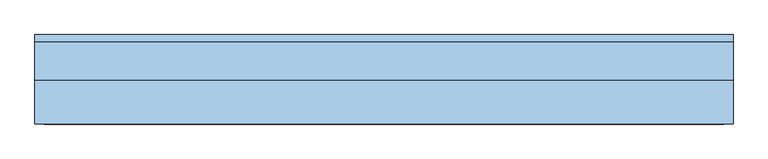
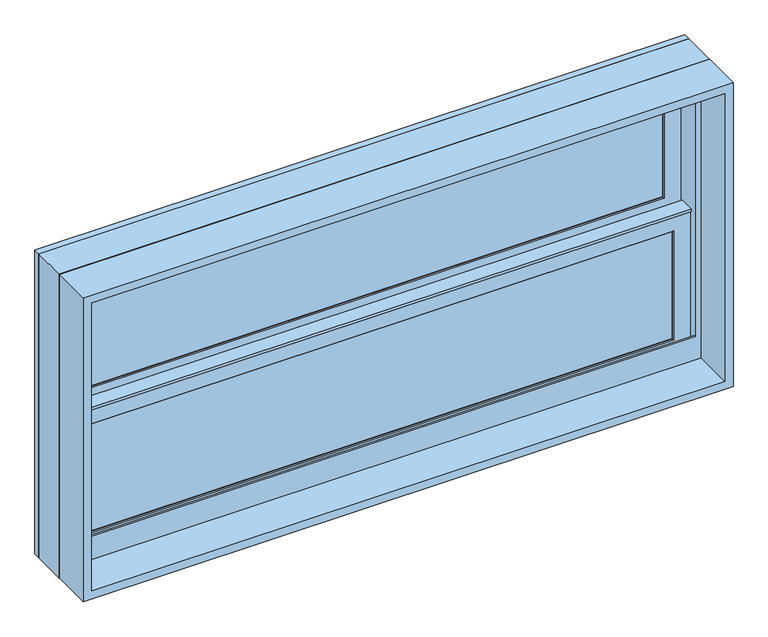
"""IFC4 building model written with IfcOpenShell, lengths in millimetres: window geometry, Window-Double_Hung-Marvin-Essential : ESDH4020."""

from ifc_helpers import new_model, si_unit, frame, origin, place, context, project, spatial, polyline, outline, extrude, faceted_brep, source, transform, mapped, element, save


def window_6a7649f0(model_context):
    return source(origin(), model_context, "Body", "SolidModel", [
        extrude(outline(polyline([(191.5583333, 20.6375), (191.5583333, 15.875), (172.5083333, 15.875), (172.5083333, 20.6375), (191.5583333, 20.6375)])), frame((0.0, 0.0, 1898.65), z_axis=(0.0, 0.0, 1.0), x_axis=(1.0, 0.0, 0.0)), (0.0, 0.0, 1.0), 222.25),
        extrude(outline(polyline([(-172.5083333, 20.6375), (-172.5083333, 15.875), (-191.5583333, 15.875), (-191.5583333, 20.6375), (-172.5083333, 20.6375)])), frame((0.0, 0.0, 1898.65), z_axis=(0.0, 0.0, 1.0), x_axis=(1.0, 0.0, 0.0)), (0.0, 0.0, 1.0), 222.25),
        extrude(outline(polyline([(546.1, 20.6375), (546.1, 15.875), (-546.1, 15.875), (-546.1, 20.6375), (546.1, 20.6375)])), frame((0.0, 0.0, 2000.25), z_axis=(0.0, 0.0, 1.0), x_axis=(1.0, 0.0, 0.0)), (0.0, 0.0, 1.0), 19.05),
        extrude(outline(polyline([(-191.5583333, 46.83125), (-191.5583333, 51.59375), (-172.5083333, 51.59375), (-172.5083333, 46.83125), (-191.5583333, 46.83125)])), frame((0.0, 0.0, 2159.0), z_axis=(0.0, 0.0, 1.0), x_axis=(1.0, 0.0, 0.0)), (0.0, 0.0, 1.0), 222.25),
        extrude(outline(polyline([(172.5083333, 46.83125), (172.5083333, 51.59375), (191.5583333, 51.59375), (191.5583333, 46.83125), (172.5083333, 46.83125)])), frame((0.0, 0.0, 2159.0), z_axis=(0.0, 0.0, 1.0), x_axis=(1.0, 0.0, 0.0)), (0.0, 0.0, 1.0), 222.25),
        extrude(outline(polyline([(-546.1, 46.83125), (-546.1, 51.59375), (546.1, 51.59375), (546.1, 46.83125), (-546.1, 46.83125)])), frame((0.0, 0.0, 2260.6), z_axis=(0.0, 0.0, 1.0), x_axis=(1.0, 0.0, 0.0)), (0.0, 0.0, 1.0), 19.05),
        extrude(outline(polyline([(191.5583333, 20.6375), (172.5083333, 20.6375), (172.5083333, 25.4), (191.5583333, 25.4), (191.5583333, 20.6375)])), frame((0.0, 0.0, 1898.65), z_axis=(0.0, 0.0, 1.0), x_axis=(1.0, 0.0, 0.0)), (0.0, 0.0, 1.0), 222.25),
        extrude(outline(polyline([(-172.5083333, 20.6375), (-191.5583333, 20.6375), (-191.5583333, 25.4), (-172.5083333, 25.4), (-172.5083333, 20.6375)])), frame((0.0, 0.0, 1898.65), z_axis=(0.0, 0.0, 1.0), x_axis=(1.0, 0.0, 0.0)), (0.0, 0.0, 1.0), 222.25),
        extrude(outline(polyline([(546.1, 20.6375), (-546.1, 20.6375), (-546.1, 25.4), (546.1, 25.4), (546.1, 20.6375)])), frame((0.0, 0.0, 2000.25), z_axis=(0.0, 0.0, 1.0), x_axis=(1.0, 0.0, 0.0)), (0.0, 0.0, 1.0), 19.05),
        extrude(outline(polyline([(-191.5583333, 56.35625), (-172.5083333, 56.35625), (-172.5083333, 51.59375), (-191.5583333, 51.59375), (-191.5583333, 56.35625)])), frame((0.0, 0.0, 2159.0), z_axis=(0.0, 0.0, 1.0), x_axis=(1.0, 0.0, 0.0)), (0.0, 0.0, 1.0), 222.25),
        extrude(outline(polyline([(172.5083333, 56.35625), (191.5583333, 56.35625), (191.5583333, 51.59375), (172.5083333, 51.59375), (172.5083333, 56.35625)])), frame((0.0, 0.0, 2159.0), z_axis=(0.0, 0.0, 1.0), x_axis=(1.0, 0.0, 0.0)), (0.0, 0.0, 1.0), 222.25),
        extrude(outline(polyline([(-546.1, 56.35625), (546.1, 56.35625), (546.1, 51.59375), (-546.1, 51.59375), (-546.1, 56.35625)])), frame((0.0, 0.0, 2260.6), z_axis=(0.0, 0.0, 1.0), x_axis=(1.0, 0.0, 0.0)), (0.0, 0.0, 1.0), 19.05),
        faceted_brep([(-573.0875, 5.6780605, 2150.9351748), (-573.0875, 5.6780605, 2146.3), (573.0875, 5.6780605, 2146.3), (573.0875, 5.6780605, 2150.9351748), (-573.0875, 34.8118605, 2150.9351748), (573.0875, 34.8118605, 2150.9351748), (573.0875, 34.8118605, 2146.3), (-573.0875, 34.8118605, 2146.3), (-573.0875, 30.1625, 2146.3), (-573.0875, 30.1625, 1871.6625), (-573.0875, 8.9241104, 1871.6625), (-573.0875, 8.9241104, 2146.3), (573.0875, 8.9241104, 2146.3), (573.0875, 30.1625, 2146.3), (573.0875, 8.9241104, 1871.6625), (573.0875, 30.1625, 1871.6625), (-557.2034752, 11.90625, 2132.0034752), (-557.2034752, 30.1625, 2132.0034752), (557.2034752, 30.1625, 2132.0034752), (557.2034752, 11.90625, 2132.0034752), (-540.54375, 10.4662439, 2115.34375), (-540.54375, 11.90625, 2115.34375), (540.54375, 11.90625, 2115.34375), (540.54375, 10.4662439, 2115.34375), (542.0858834, 8.9241104, 2116.8858834), (-542.0858834, 8.9241104, 2116.8858834), (557.2034752, 30.1625, 1887.5465248), (557.2034752, 11.90625, 1887.5465248), (540.54375, 11.90625, 1904.20625), (540.54375, 10.4662439, 1904.20625), (542.0858834, 8.9241104, 1902.6641166), (-557.2034752, 30.1625, 1887.5465248), (-557.2034752, 11.90625, 1887.5465248), (-540.54375, 11.90625, 1904.20625), (-540.54375, 10.4662439, 1904.20625), (-542.0858834, 8.9241104, 1902.6641166)], [[[0, 1, 2, 3]], [[4, 5, 6, 7]], [[1, 0, 4, 7, 8, 9, 10, 11]], [[2, 1, 11, 12]], [[7, 6, 13, 8]], [[3, 2, 12, 14, 15, 13, 6, 5]], [[0, 3, 5, 4]], [[16, 17, 18, 19]], [[20, 21, 22, 23]], [[20, 23, 24, 25]], [[19, 18, 26, 27]], [[23, 22, 28, 29]], [[24, 23, 29, 30]], [[27, 26, 31, 32]], [[29, 28, 33, 34]], [[30, 29, 34, 35]], [[15, 14, 10, 9]], [[15, 9, 8, 13], [18, 17, 31, 26]], [[17, 16, 32, 31]], [[16, 19, 27, 32], [22, 21, 33, 28]], [[21, 20, 34, 33]], [[20, 25, 35, 34]], [[10, 14, 12, 11], [25, 24, 30, 35]]]),
        extrude(outline(polyline([(38.5955581, 2132.0125), (33.5778968, 2132.0125), (33.5778968, 2133.6), (39.9405976, 2133.6), (39.9405976, 2132.0125), (61.515625, 2132.0125), (47.6307501, 2128.6975159), (38.5955581, 2128.6975159), (38.5955581, 2132.0125)])), frame((-573.0875, 0.0, 0.0), z_axis=(1.0, 0.0, 0.0), x_axis=(0.0, 1.0, 0.0)), (0.0, 0.0, 1.0), 1146.175),
        faceted_brep([(603.25, 0.0, 1841.5), (603.25, 0.0, 2438.4), (-603.25, 0.0, 2438.4), (-603.25, 0.0, 1841.5), (577.05625, 0.0, 1902.61875), (-577.05625, 0.0, 1902.61875), (-577.05625, 0.0, 2412.20625), (577.05625, 0.0, 2412.20625), (577.05625, 3.96875, 1841.5), (-577.05625, 3.96875, 1841.5), (-577.05625, 3.96875, 1902.61875), (577.05625, 3.96875, 1902.61875), (-603.25, 65.6828125, 1841.5), (-577.05625, 65.6828125, 1841.5), (577.05625, 65.6828125, 1841.5), (603.25, 65.6828125, 1841.5), (-603.25, 65.6828125, 2438.4), (603.25, 65.6828125, 2438.4), (577.05625, 65.6828125, 2412.20625), (-577.05625, 65.6828125, 2412.20625)], [[[0, 1, 2, 3], [4, 5, 6, 7]], [[8, 9, 10, 11]], [[5, 4, 11, 10]], [[0, 3, 12, 13, 9, 8, 14, 15]], [[13, 12, 16, 17, 15, 14, 18, 19]], [[13, 19, 6, 5, 10, 9]], [[7, 6, 19, 18]], [[18, 14, 8, 11, 4, 7]], [[1, 0, 15, 17]], [[2, 1, 17, 16]], [[3, 2, 16, 12]]]),
        faceted_brep([(577.05625, 30.1625, 2139.95), (575.46875, 30.1625, 2139.95), (575.46875, 30.1625, 1865.8544613), (577.05625, 30.1625, 1865.8544613), (-575.46875, 30.1625, 2139.95), (-577.05625, 30.1625, 2139.95), (-577.05625, 30.1625, 1865.8544613), (-575.46875, 30.1625, 1865.8544613), (575.46875, 63.5, 2139.95), (577.05625, 63.5, 2139.95), (577.05625, 63.5, 1859.3743077), (575.46875, 63.5, 1859.3743077), (-577.05625, 63.5, 2139.95), (-575.46875, 63.5, 2139.95), (-575.46875, 63.5, 1859.3743077), (-577.05625, 63.5, 1859.3743077), (588.3108932, 3.96875, 1870.9460105), (588.3108932, 3.96875, 1841.5), (588.3108932, 65.6828125, 1841.5), (588.3108932, 65.6828125, 1858.950012), (-588.3108932, 3.96875, 1841.5), (-588.3108932, 3.96875, 1870.9460105), (-588.3108932, 65.6828125, 1858.950012), (-588.3108932, 65.6828125, 1841.5), (588.3108932, 78.58125, 1856.4428097), (-588.3108932, 78.58125, 1856.4428097), (-586.2971252, 68.2348864, 1858.4539391), (-568.33135, 68.2348864, 1858.4539391), (-568.33135, 65.6828125, 1858.950012), (568.33135, 65.6828125, 1858.950012), (568.33135, 68.2348864, 1858.4539391), (586.2971252, 68.2348864, 1858.4539391), (-603.25, 65.6828125, 1841.5), (-603.25, 78.5948249, 1841.5), (603.25, 78.5948249, 1841.5), (603.25, 65.6828125, 1841.5), (-603.25, 78.58125, 2438.4), (603.25, 78.58125, 2438.4), (588.3108932, 78.58125, 2423.4608932), (-588.3108932, 78.58125, 2423.4608932), (-603.25, 65.6828125, 2438.4), (-586.2971252, 68.2348864, 2421.4471252), (586.2971252, 68.2348864, 2421.4471252), (568.33135, 68.2348864, 2403.48135), (-568.33135, 68.2348864, 2403.48135), (-568.33135, 65.6828125, 2403.48135), (568.33135, 65.6828125, 2403.48135), (603.25, 65.6828125, 2438.4)], [[[0, 1, 2, 3]], [[4, 5, 6, 7]], [[8, 9, 10, 11]], [[12, 13, 14, 15]], [[1, 8, 11, 2]], [[9, 0, 3, 10]], [[1, 0, 9, 8]], [[5, 4, 13, 12]], [[5, 12, 15, 6]], [[13, 4, 7, 14]], [[16, 17, 18, 19]], [[20, 21, 22, 23]], [[24, 25, 26, 27, 28, 22, 21, 16, 19, 29, 30, 31], [3, 2, 11, 10], [7, 6, 15, 14]], [[17, 16, 21, 20]], [[17, 20, 23, 32, 33, 34, 35, 18]], [[34, 33, 36, 37], [25, 24, 38, 39]], [[33, 32, 40, 36]], [[39, 41, 26, 25]], [[41, 42, 31, 30, 43, 44, 27, 26]], [[44, 45, 28, 27]], [[40, 32, 23, 22, 28, 45, 46, 29, 19, 18, 35, 47]], [[36, 40, 47, 37]], [[39, 38, 42, 41]], [[44, 43, 46, 45]], [[34, 37, 47, 35]], [[42, 38, 24, 31]], [[46, 43, 30, 29]]]),
        extrude(outline(polyline([(553.24375, 11.90625), (-553.24375, 11.90625), (-553.24375, 15.08125), (553.24375, 15.08125), (553.24375, 11.90625)])), frame((0.0, 0.0, 1891.50625), z_axis=(0.0, 0.0, 1.0), x_axis=(1.0, 0.0, 0.0)), (0.0, 0.0, 1.0), 236.5375),
        extrude(outline(polyline([(553.24375, 42.8625), (-553.24375, 42.8625), (-553.24375, 46.0375), (553.24375, 46.0375), (553.24375, 42.8625)])), frame((0.0, 0.0, 2151.85625), z_axis=(0.0, 0.0, 1.0), x_axis=(1.0, 0.0, 0.0)), (0.0, 0.0, 1.0), 236.5375),
        faceted_brep([(-540.54375, 31.194477, 2115.34375), (-542.0858834, 32.7366104, 2116.8858834), (542.0858834, 32.7366104, 2116.8858834), (540.54375, 31.194477, 2115.34375), (-540.54375, 30.1625, 2115.34375), (540.54375, 30.1625, 2115.34375), (-573.0875, 32.7366104, 2147.8875), (-573.0875, 30.1625, 2147.8875), (573.0875, 30.1625, 2147.8875), (573.0875, 32.7366104, 2147.8875), (542.0858834, 32.7366104, 1902.6641166), (540.54375, 31.194477, 1904.20625), (540.54375, 30.1625, 1904.20625), (573.0875, 30.1625, 1871.6625), (573.0875, 32.7366104, 1871.6625), (-542.0858834, 32.7366104, 1902.6641166), (-540.54375, 31.194477, 1904.20625), (-540.54375, 30.1625, 1904.20625), (-573.0875, 30.1625, 1871.6625), (-573.0875, 32.7366104, 1871.6625)], [[[0, 1, 2, 3]], [[4, 0, 3, 5]], [[6, 7, 8, 9]], [[3, 2, 10, 11]], [[5, 3, 11, 12]], [[9, 8, 13, 14]], [[11, 10, 15, 16]], [[12, 11, 16, 17]], [[14, 13, 18, 19]], [[9, 14, 19, 6], [1, 15, 10, 2]], [[16, 15, 1, 0]], [[17, 16, 0, 4]], [[7, 18, 13, 8], [5, 12, 17, 4]], [[19, 18, 7, 6]]]),
        faceted_brep([(-557.2034752, 42.8625, 2392.3534752), (-557.2034752, 61.11875, 2392.3534752), (557.2034752, 61.11875, 2392.3534752), (557.2034752, 42.8625, 2392.3534752), (-540.54375, 41.4224939, 2375.69375), (-540.54375, 42.8625, 2375.69375), (540.54375, 42.8625, 2375.69375), (540.54375, 41.4224939, 2375.69375), (-542.0858834, 39.8803604, 2377.2358834), (542.0858834, 39.8803604, 2377.2358834), (-573.0875, 61.11875, 2408.2375), (-573.0875, 39.8803604, 2408.2375), (573.0875, 39.8803604, 2408.2375), (573.0875, 61.11875, 2408.2375), (557.2034752, 61.11875, 2147.8965248), (557.2034752, 42.8625, 2147.8965248), (540.54375, 42.8625, 2164.55625), (540.54375, 41.4224939, 2164.55625), (542.0858834, 39.8803604, 2163.0141166), (573.0875, 39.8803604, 2132.0125), (573.0875, 61.11875, 2132.0125), (-557.2034752, 61.11875, 2147.8965248), (-557.2034752, 42.8625, 2147.8965248), (-540.54375, 42.8625, 2164.55625), (-540.54375, 41.4224939, 2164.55625), (-542.0858834, 39.8803604, 2163.0141166), (-573.0875, 39.8803604, 2132.0125), (-573.0875, 61.11875, 2132.0125)], [[[0, 1, 2, 3]], [[4, 5, 6, 7]], [[8, 4, 7, 9]], [[10, 11, 12, 13]], [[3, 2, 14, 15]], [[7, 6, 16, 17]], [[9, 7, 17, 18]], [[13, 12, 19, 20]], [[15, 14, 21, 22]], [[17, 16, 23, 24]], [[18, 17, 24, 25]], [[20, 19, 26, 27]], [[13, 20, 27, 10], [1, 21, 14, 2]], [[22, 21, 1, 0]], [[3, 15, 22, 0], [5, 23, 16, 6]], [[24, 23, 5, 4]], [[25, 24, 4, 8]], [[11, 26, 19, 12], [9, 18, 25, 8]], [[27, 26, 11, 10]]]),
        faceted_brep([(-573.0875, 61.11875, 2132.0125), (-573.0875, 63.6928604, 2132.0125), (573.0875, 63.6928604, 2132.0125), (573.0875, 61.11875, 2132.0125), (-540.54375, 62.150727, 2164.55625), (-540.54375, 61.11875, 2164.55625), (540.54375, 61.11875, 2164.55625), (540.54375, 62.150727, 2164.55625), (-542.0858834, 63.6928604, 2163.0141166), (542.0858834, 63.6928604, 2163.0141166), (573.0875, 63.6928604, 2408.2375), (573.0875, 61.11875, 2408.2375), (540.54375, 61.11875, 2375.69375), (540.54375, 62.150727, 2375.69375), (542.0858834, 63.6928604, 2377.2358834), (-573.0875, 63.6928604, 2408.2375), (-573.0875, 61.11875, 2408.2375), (-540.54375, 61.11875, 2375.69375), (-540.54375, 62.150727, 2375.69375), (-542.0858834, 63.6928604, 2377.2358834)], [[[0, 1, 2, 3]], [[4, 5, 6, 7]], [[8, 4, 7, 9]], [[3, 2, 10, 11]], [[7, 6, 12, 13]], [[9, 7, 13, 14]], [[11, 10, 15, 16]], [[13, 12, 17, 18]], [[14, 13, 18, 19]], [[16, 15, 1, 0]], [[3, 11, 16, 0], [5, 17, 12, 6]], [[18, 17, 5, 4]], [[19, 18, 4, 8]], [[1, 15, 10, 2], [9, 14, 19, 8]]]),
        extrude(outline(polyline([(553.24375, 26.19375), (-553.24375, 26.19375), (-553.24375, 30.1625), (553.24375, 30.1625), (553.24375, 26.19375)])), frame((0.0, 0.0, 1891.50625), z_axis=(0.0, 0.0, 1.0), x_axis=(1.0, 0.0, 0.0)), (0.0, 0.0, 1.0), 236.5375),
        extrude(outline(polyline([(553.24375, 57.15), (-553.24375, 57.15), (-553.24375, 61.11875), (553.24375, 61.11875), (553.24375, 57.15)])), frame((0.0, 0.0, 2151.85625), z_axis=(0.0, 0.0, 1.0), x_axis=(1.0, 0.0, 0.0)), (0.0, 0.0, 1.0), 236.5375),
        extrude(outline(polyline([(2438.4, 603.25), (2438.4, -603.25), (1841.5, -603.25), (1841.5, 603.25), (2438.4, 603.25)]), holes=[polyline([(2422.525, 587.375), (1857.375, 587.375), (1857.375, -587.375), (2422.525, -587.375), (2422.525, 587.375)])]), frame((0.0, -76.2, 0.0), z_axis=(0.0, 1.0, 0.0), x_axis=(0.0, 0.0, 1.0)), (0.0, 0.0, 1.0), 75.40625),
    ])


if __name__ == "__main__":
    model = new_model("IFC4")
    model_context = context("Model", 3, world=origin())
    ifc_project = project(units=[si_unit("LENGTHUNIT", "METRE", prefix="MILLI")], contexts=[model_context])
    site = spatial("IfcSite", under=ifc_project)
    building = spatial("IfcBuilding", under=site)
    placement = place(None, origin())
    window_shape = window_6a7649f0(model_context)
    element("IfcWindow", 1, ObjectType="Window-Double_Hung-Marvin-Essential : ESDH4020", at=placement, inside=building, context=model_context, shape_type="MappedRepresentation", body=[
        mapped(window_shape, transform((0.0, 0.0, 0.0), x_axis=(1.0, 0.0, 0.0), y_axis=(0.0, 1.0, 0.0), z_axis=(0.0, 0.0, 1.0))),
    ])
    save(model, "model.ifc")

# Revit data of these elements
# Type "Window-Double_Hung-Marvin-Essential : ESDH4020"
#   Type Mark = "25"
#   Window Type = "Essential Double Hung"
#   Product data url = "https://bimobject.com/marvin-windows-and-doors/product/marvin-dhwau"
#   Product Guid = "c4a96547-874c-4385-91dc-a058adc19d98"
#   Frame = "All Ultrex"
#   Egress Window = "No"
#   URL = "www.marvin.com"
#   Model = "ESDH4020"
#   Manufacturer = "Marvin Windows and Doors"
#   Label Egress = ""
#   Glass Type = "IG Low E II with Argon"
#   Design Pressure = "DP50"
#   Description = "4824 DBHG"
#   Analytic Construction = "<None>"
#   Prairie Corner Width = 0' - 4"
#   Prairie Corner Height = 0' - 4"
#   Egress Width = 3' - 8 9/16"
#   Egress Height = 0' - 7 27/128"
#   Rough Width = 4' - 0"
#   Rough Height = 2' - 0"
#   Nominal Width = 4' - 0"
#   Nominal Height = 2' - 0"
#   Inset to Installation Flange [instance default] = 0' - 1"
#   Height = 1' - 11 1/2"
#   Egress Area = 2.23151 SF
#   Default Head Height = 8' - 0"
#   Width = 3' - 11 1/2"
#   Daylight Area = 4.9139 SF
#   DLO Width = 3' - 6 9/16"
#   DLO Height = 0' - 8 5/16"
#   Muntins Top Sash = yes
#   Lites Wide Top Sash = 3
#   Lites Wide Bottom Sash = 3
#   Lites High Top Sash = 2
#   Lites High Bottom Sash = 2
#   Lite Cut Prairie 9 = no
#   Lite Cut HV Grid = yes
#   Muntins Bottom Sash = yes
#   Label Visibility = no
#   Jamb Extension Visibility = yes
#   Edition number = 1
#   Interior Material = Ultrex-Marvin-Stonewhite
#   Glazing Material = Glass-Marvin-IG Low E II with Argon
#   Cladding Material = Ultrex-Marvin-Pebblegray
#   Wall Closure = (empty or 0)
#   Assembly Code = ""
# Element 1 (IfcWindow, "Window-Double_Hung-Marvin-Essential : ESDH4020")
#   Materials on its faces: "Ultrex-Marvin-Pebblegray", "Ultrex-Marvin-Stonewhite", "Glass-Marvin-IG Low E II with Argon"
# Materials
#   "Ultrex-Marvin-Stonewhite": class "Paint", colour RGB 250 251 245, transparency 0
#   "Glass-Marvin-IG Low E II with Argon": class "Glass", colour RGB 0 128 192, transparency 0.85
#   "Ultrex-Marvin-Pebblegray": class "Paint", colour RGB 189 185 173, transparency 0
